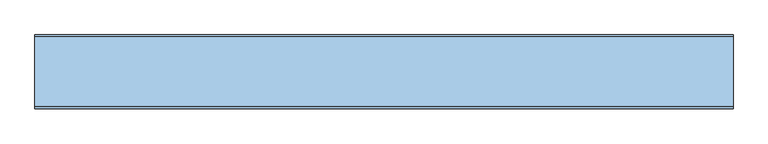
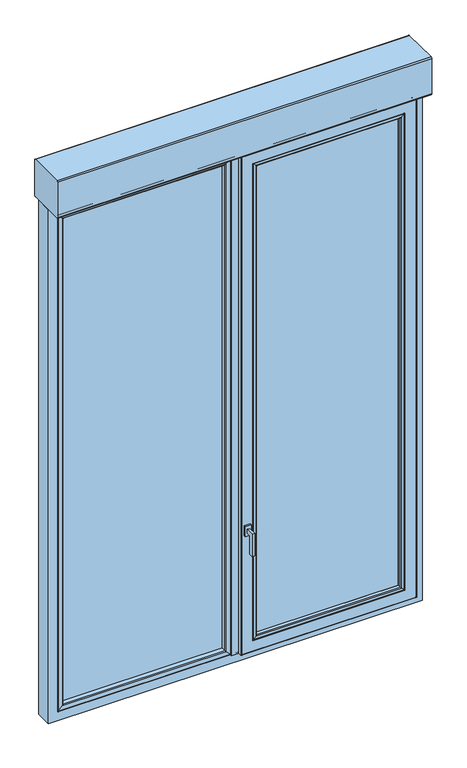
"""IFC4 building model written with IfcOpenShell, lengths in millimetres: window geometry, 2019_ES_Ventana_Replus_re80pvc301_11103_box_1-Hoja_Panel-Fijo-Lateral_con-Compacto : Salla."""

from ifc_helpers import new_model, si_unit, point, frame, frame_2d, origin, place, context, project, spatial, polyline, circle_curve, ellipse_curve, trimmed, segment, composite_curve, outline, extrude, source, transform, mapped, element, save
from ifc_brep_helpers import plane_surface, cylinder_surface, advanced_brep


def window_06f9a558(model_context):
    return source(origin(), model_context, "Body", "SolidModel", [
        extrude(outline(composite_curve([segment(polyline([(55.0, 3355.0), (-120.0, 3355.0)]), True, "CONTINUOUS"), segment(trimmed(circle_curve(frame_2d((-120.0, 3360.0)), 5.0), [point((-120.0, 3355.0))], [point((-125.0, 3360.0))], False, "CARTESIAN"), True, "CONTINUOUS"), segment(polyline([(-125.0, 3360.0), (-125.0, 3535.0)]), True, "CONTINUOUS"), segment(trimmed(circle_curve(frame_2d((-120.0, 3535.0)), 5.0), [point((-125.0, 3535.0))], [point((-120.0, 3540.0))], False, "CARTESIAN"), True, "CONTINUOUS"), segment(polyline([(-120.0, 3540.0), (55.0, 3540.0)]), True, "CONTINUOUS"), segment(trimmed(circle_curve(frame_2d((55.0, 3535.0)), 5.0), [point((55.0, 3540.0))], [point((60.0, 3535.0))], False, "CARTESIAN"), True, "CONTINUOUS"), segment(polyline([(60.0, 3535.0), (60.0, 3360.0)]), True, "CONTINUOUS"), segment(trimmed(circle_curve(frame_2d((55.0, 3360.0)), 5.0), [point((60.0, 3360.0))], [point((55.0, 3355.0))], False, "CARTESIAN"), True, "CONTINUOUS")], self_intersect=False)), frame((-875.0, 0.0, 0.0), z_axis=(1.0, 0.0, 0.0), x_axis=(0.0, 1.0, 0.0)), (0.0, 0.0, 1.0), 1750.0),
        extrude(outline(polyline([(-78.4999991, 1470.0), (-78.4999991, 1450.0), (-98.4999991, 1450.0), (-98.4999991, 1360.0), (-118.4999991, 1360.0), (-118.4999991, 1470.0), (-78.4999991, 1470.0)])), frame((38.5, 0.0, 0.0), z_axis=(1.0, 0.0, 0.0), x_axis=(0.0, 1.0, 0.0)), (0.0, 0.0, 1.0), 12.0),
        extrude(outline(polyline([(58.7312385, -78.4999991), (30.2687615, -78.4999991), (30.2687615, -68.4999991), (58.7312385, -68.4999991), (58.7312385, -78.4999991)])), frame((0.0, 0.0, 1435.217127), z_axis=(0.0, 0.0, 1.0), x_axis=(1.0, 0.0, 0.0)), (0.0, 0.0, 1.0), 49.565746),
        extrude(outline(polyline([(-37.0063666, 11.4999962), (-37.0063666, 7.4999962), (-809.1891471, 7.4999962), (-809.1891471, 11.4999962), (-37.0063666, 11.4999962)])), frame((0.0, 0.0, 875.6108529), z_axis=(0.0, 0.0, 1.0), x_axis=(1.0, 0.0, 0.0)), (0.0, 0.0, 1.0), 2413.7782941),
        extrude(outline(polyline([(-37.0063666, -6.5), (-37.0063666, -10.5), (-809.1891471, -10.5), (-809.1891471, -6.5), (-37.0063666, -6.5)])), frame((0.0, 0.0, 875.6108529), z_axis=(0.0, 0.0, 1.0), x_axis=(1.0, 0.0, 0.0)), (0.0, 0.0, 1.0), 2413.7782941),
        extrude(outline(polyline([(-37.0063666, -24.4999997), (-37.0063666, -28.4999997), (-809.1891471, -28.4999997), (-809.1891471, -24.4999997), (-37.0063666, -24.4999997)])), frame((0.0, 0.0, 875.6108529), z_axis=(0.0, 0.0, 1.0), x_axis=(1.0, 0.0, 0.0)), (0.0, 0.0, 1.0), 2413.7782941),
        advanced_brep(
        [(-22.1502489, -49.9816666, 3309.0497511), (-41.8192398, -49.2838062, 3289.3807602), (-41.8192398, -49.2838062, 875.6192398), (-22.1502489, -49.9816666, 855.9502489), (-46.4697163, -45.5846502, 3284.7302837), (-46.4697163, -45.5846502, 880.2697163), (-809.3807594, -49.2838062, 875.6192398), (-829.0497503, -49.9816666, 855.9502489), (-21.0, -48.871505, 3310.2), (-21.0, -48.871505, 854.8), (-51.0475336, -28.5000036, 3280.1524664), (-51.0475336, -28.5000036, 884.8475336), (-804.7302829, -45.5846502, 880.2697163), (-43.2922784, -28.5000036, 877.0922784), (-807.9077208, -28.5000036, 877.0922784), (-807.9077208, -28.5000036, 3287.9077216), (-43.2922784, -28.5000036, 3287.9077216), (-800.1524657, -28.5000036, 3280.1524664), (-800.1524657, -28.5000036, 884.8475336), (-35.4855, -36.306782, 3295.7145), (-35.4855, -36.306782, 869.2855), (-35.4855, -39.5069121, 3295.7145), (-35.4855, -39.5069121, 869.2855), (-815.7144993, -36.306782, 869.2855), (-21.0, -39.5069121, 854.8), (-830.1999993, -39.5069121, 854.8), (-830.1999993, -39.5069121, 3310.2), (-21.0, -39.5069121, 3310.2), (-815.7144993, -39.5069121, 3295.7145), (-815.7144993, -39.5069121, 869.2855), (-830.1999993, -48.871505, 854.8), (-809.3807594, -49.2838062, 3289.3807602), (-829.0497503, -49.9816666, 3309.0497511), (-804.7302829, -45.5846502, 3284.7302837), (-815.7144993, -36.306782, 3295.7145), (-830.1999993, -48.871505, 3310.2)],
        [
            (0, 1),
            (1, 2),
            (2, 3),
            (3, 0),
            (1, 4, ellipse_curve(frame((-41.6449168, -44.2918491, 3289.5550832), z_axis=(0.7071067811865475, 0.0, -0.7071067811865475), x_axis=(0.7071067811865474, 0.0, 0.7071067811865476)), 7.0639967, 4.995)),
            (4, 5),
            (5, 2, ellipse_curve(frame((-41.6449168, -44.2918491, 875.4449168), z_axis=(0.7071067811865475, 0.0, 0.7071067811865475), x_axis=(-0.7071067811865474, 0.0, 0.7071067811865476)), 7.0639967, 4.995)),
            (2, 6),
            (6, 7),
            (7, 3),
            (8, 0, ellipse_curve(frame((-22.1108601, -48.871505, 3309.0891399), z_axis=(0.7071067811865475, 0.0, -0.7071067811865475), x_axis=(0.7071067811865474, 0.0, 0.7071067811865476)), 1.5709935, 1.1108601)),
            (3, 9, ellipse_curve(frame((-22.1108601, -48.871505, 855.9108601), z_axis=(0.7071067811865475, 0.0, 0.7071067811865475), x_axis=(-0.7071067811865474, 0.0, 0.7071067811865476)), 1.5709935, 1.1108601)),
            (9, 8),
            (4, 10),
            (10, 11),
            (11, 5),
            (5, 12),
            (12, 6, ellipse_curve(frame((-809.5550824, -44.2918491, 875.4449168), z_axis=(0.7071067811865475, 0.0, -0.7071067811865475), x_axis=(0.7071067811865476, 0.0, 0.7071067811865474)), 7.0639967, 4.995)),
            (13, 14),
            (14, 15),
            (15, 16),
            (16, 13),
            (10, 17),
            (17, 18),
            (18, 11),
            (18, 12),
            (16, 19),
            (19, 20),
            (20, 13),
            (19, 21),
            (21, 22),
            (22, 20),
            (20, 23),
            (23, 14),
            (24, 25),
            (25, 26),
            (26, 27),
            (27, 24),
            (21, 28),
            (28, 29),
            (29, 22),
            (29, 23),
            (9, 24),
            (27, 8),
            (9, 30),
            (30, 25),
            (7, 30, ellipse_curve(frame((-829.0891391, -48.871505, 855.9108601), z_axis=(0.7071067811865475, 0.0, -0.7071067811865475), x_axis=(0.7071067811865476, 0.0, 0.7071067811865474)), 1.5709935, 1.1108601)),
            (6, 31),
            (31, 32),
            (32, 7),
            (12, 33),
            (33, 31, ellipse_curve(frame((-809.5550824, -44.2918491, 3289.5550832), z_axis=(-0.7071067811865475, 0.0, -0.7071067811865475), x_axis=(0.7071067811865474, 0.0, -0.7071067811865476)), 7.0639967, 4.995)),
            (17, 33),
            (23, 34),
            (34, 15),
            (28, 34),
            (30, 35),
            (35, 26),
            (32, 35, ellipse_curve(frame((-829.0891391, -48.871505, 3309.0891399), z_axis=(-0.7071067811865475, 0.0, -0.7071067811865475), x_axis=(0.7071067811865474, 0.0, -0.7071067811865476)), 1.5709935, 1.1108601)),
            (31, 1),
            (0, 32),
            (33, 4),
            (34, 19),
            (35, 8),
        ],
        [
            plane_surface(frame((-41.8192398, -49.2838062, 3289.3807602), z_axis=(-0.03545791932093311, -0.9993711702652975, 0.0), x_axis=(0.0, 0.0, -1.0))),
            cylinder_surface(frame((-41.6449168, -44.2918491, 3317.2), z_axis=(0.0, 0.0, 1.0), x_axis=(-1.0, 0.0, 0.0)), 4.995),
            plane_surface(frame((-41.8192398, -49.2838062, 875.6192398), z_axis=(0.0, -0.9993711702652976, 0.035457919320929884), x_axis=(-1.0, 0.0, 0.0))),
            cylinder_surface(frame((-22.1108601, -48.871505, 3317.2), z_axis=(0.0, 0.0, 1.0), x_axis=(-1.0, 0.0, 0.0)), 1.1108601),
            plane_surface(frame((-51.0475336, -28.5000036, 3280.1524664), z_axis=(-0.9659258262890619, -0.25881904510254483, 0.0), x_axis=(0.0, 0.0, -1.0))),
            cylinder_surface(frame((-14.0, -44.2918491, 875.4449168), z_axis=(1.0, 0.0, 0.0), x_axis=(0.0, 0.0, 1.0)), 4.995),
            plane_surface(frame((-807.9077208, -28.5000036, 3287.9077216), z_axis=(0.0, 1.0, 0.0), x_axis=(1.0, 0.0, 0.0))),
            plane_surface(frame((-51.0475336, -28.5000036, 884.8475336), z_axis=(0.0, -0.25881904510254794, 0.965925826289061), x_axis=(-1.0, 0.0, 0.0))),
            plane_surface(frame((-35.4855, -36.306782, 3295.7145), z_axis=(0.7071067811865617, 0.7071067811865334, 0.0), x_axis=(0.0, 0.0, -1.0))),
            plane_surface(frame((-35.4855, -39.5069121, 3295.7145), z_axis=(1.0, 0.0, 0.0), x_axis=(0.0, 0.0, -1.0))),
            plane_surface(frame((-35.4855, -36.306782, 869.2855), z_axis=(0.0, 0.7071067811865357, -0.7071067811865593), x_axis=(-1.0, 0.0, 0.0))),
            plane_surface(frame((-830.1999993, -39.5069121, 3310.2), z_axis=(0.0, 1.0, 0.0), x_axis=(1.0, 0.0, 0.0))),
            plane_surface(frame((-35.4855, -39.5069121, 869.2855), z_axis=(0.0, 0.0, -1.0), x_axis=(-1.0, 0.0, 0.0))),
            plane_surface(frame((-21.0, -46.2002121, 3310.2), z_axis=(1.0, 0.0, 0.0), x_axis=(0.0, 0.0, -1.0))),
            plane_surface(frame((-21.0, -46.2002121, 854.8), z_axis=(0.0, 0.0, -1.0), x_axis=(-1.0, 0.0, 0.0))),
            cylinder_surface(frame((-14.0, -48.871505, 855.9108601), z_axis=(1.0, 0.0, 0.0), x_axis=(0.0, 0.0, 1.0)), 1.1108601),
            plane_surface(frame((-809.3807594, -49.2838062, 875.6192398), z_axis=(0.03545791932092666, -0.9993711702652978, 0.0), x_axis=(0.0, 0.0, 1.0))),
            cylinder_surface(frame((-809.5550824, -44.2918491, 847.8), z_axis=(0.0, 0.0, -1.0), x_axis=(1.0, 0.0, 0.0)), 4.995),
            plane_surface(frame((-800.1524657, -28.5000036, 884.8475336), z_axis=(0.9659258262890602, -0.2588190451025511, 0.0), x_axis=(0.0, 0.0, 1.0))),
            plane_surface(frame((-815.7144993, -36.306782, 869.2855), z_axis=(-0.707106781186557, 0.707106781186538, 0.0), x_axis=(0.0, 0.0, 1.0))),
            plane_surface(frame((-815.7144993, -39.5069121, 869.2855), z_axis=(-1.0, 0.0, 0.0), x_axis=(0.0, 0.0, 1.0))),
            plane_surface(frame((-830.1999993, -46.2002121, 854.8), z_axis=(-1.0, 0.0, 0.0), x_axis=(0.0, 0.0, 1.0))),
            cylinder_surface(frame((-829.0891391, -48.871505, 847.8), z_axis=(0.0, 0.0, -1.0), x_axis=(1.0, 0.0, 0.0)), 1.1108601),
            plane_surface(frame((-809.3807594, -49.2838062, 3289.3807602), z_axis=(0.0, -0.9993711702652976, -0.035457919320929884), x_axis=(1.0, 0.0, 0.0))),
            cylinder_surface(frame((-837.1999993, -44.2918491, 3289.5550832), z_axis=(-1.0, 0.0, 0.0), x_axis=(0.0, 0.0, -1.0)), 4.995),
            plane_surface(frame((-800.1524657, -28.5000036, 3280.1524664), z_axis=(0.0, -0.258819045102548, -0.9659258262890611), x_axis=(1.0, 0.0, 0.0))),
            plane_surface(frame((-815.7144993, -36.306782, 3295.7145), z_axis=(0.0, 0.7071067811865357, 0.7071067811865593), x_axis=(1.0, 0.0, 0.0))),
            plane_surface(frame((-815.7144993, -39.5069121, 3295.7145), z_axis=(0.0, 0.0, 1.0), x_axis=(1.0, 0.0, 0.0))),
            plane_surface(frame((-830.1999993, -46.2002121, 3310.2), z_axis=(0.0, 0.0, 1.0), x_axis=(1.0, 0.0, 0.0))),
            cylinder_surface(frame((-837.1999993, -48.871505, 3309.0891399), z_axis=(-1.0, 0.0, 0.0), x_axis=(0.0, 0.0, -1.0)), 1.1108601),
        ],
        [
            (0, [[1, 2, 3, 4]]),
            (1, [[5, 6, 7, -2]]),
            (2, [[-3, 8, 9, 10]]),
            (3, [[11, -4, 12, 13]]),
            (4, [[14, 15, 16, -6]]),
            (5, [[-7, 17, 18, -8]]),
            (6, [[19, 20, 21, 22], [23, 24, 25, -15]]),
            (7, [[-16, -25, 26, -17]]),
            (8, [[27, 28, 29, -22]]),
            (9, [[30, 31, 32, -28]]),
            (10, [[-29, 33, 34, -19]]),
            (11, [[35, 36, 37, 38], [39, 40, 41, -31]]),
            (12, [[-32, -41, 42, -33]]),
            (13, [[-13, 43, -38, 44]]),
            (14, [[-43, 45, 46, -35]]),
            (15, [[-12, -10, 47, -45]]),
            (16, [[-9, 48, 49, 50]]),
            (17, [[-18, 51, 52, -48]]),
            (18, [[-26, -24, 53, -51]]),
            (19, [[-34, 54, 55, -20]]),
            (20, [[-42, -40, 56, -54]]),
            (21, [[-46, 57, 58, -36]]),
            (22, [[-47, -50, 59, -57]]),
            (23, [[-49, 60, -1, 61]]),
            (24, [[-52, 62, -5, -60]]),
            (25, [[-53, -23, -14, -62]]),
            (26, [[-55, 63, -27, -21]]),
            (27, [[-56, -39, -30, -63]]),
            (28, [[-58, 64, -44, -37]]),
            (29, [[-59, -61, -11, -64]]),
        ],
    ),
        extrude(outline(polyline([(3252.0, 772.1999993), (3252.0, 81.0), (912.8, 81.0), (912.8, 772.1999993), (3252.0, 772.1999993)]), holes=[polyline([(920.8, 764.1999993), (920.8, 89.0), (3244.0, 89.0), (3244.0, 764.1999993), (920.8, 764.1999993)])]), frame((0.0, -27.0000002, 0.0), z_axis=(0.0, 1.0, 0.0), x_axis=(0.0, 0.0, 1.0)), (0.0, 0.0, 1.0), 16.0000002),
        extrude(outline(polyline([(3252.0, 772.1999993), (3252.0, 81.0), (912.8, 81.0), (912.8, 772.1999993), (3252.0, 772.1999993)]), holes=[polyline([(920.8, 764.1999993), (920.8, 89.0), (3244.0, 89.0), (3244.0, 764.1999993), (920.8, 764.1999993)])]), frame((0.0, -47.0000002, 0.0), z_axis=(0.0, 1.0, 0.0), x_axis=(0.0, 0.0, 1.0)), (0.0, 0.0, 1.0), 16.0000002),
        extrude(outline(polyline([(3283.3891471, -43.0063666), (3283.3891471, -803.1891471), (881.8608529, -803.1891471), (881.8608529, -43.0063666), (3283.3891471, -43.0063666)]), holes=[polyline([(889.8608529, -51.0063666), (889.8608529, -795.1891471), (3275.3891471, -795.1891471), (3275.3891471, -51.0063666), (889.8608529, -51.0063666)])]), frame((0.0, -24.5, 0.0), z_axis=(0.0, 1.0, 0.0), x_axis=(0.0, 0.0, 1.0)), (0.0, 0.0, 1.0), 14.0),
        extrude(outline(polyline([(3283.3891471, -43.0063666), (3283.3891471, -803.1891471), (881.8608529, -803.1891471), (881.8608529, -43.0063666), (3283.3891471, -43.0063666)]), holes=[polyline([(889.8608529, -51.0063666), (889.8608529, -795.1891471), (3275.3891471, -795.1891471), (3275.3891471, -51.0063666), (889.8608529, -51.0063666)])]), frame((0.0, -6.5, 0.0), z_axis=(0.0, 1.0, 0.0), x_axis=(0.0, 0.0, 1.0)), (0.0, 0.0, 1.0), 14.0),
        advanced_brep(
        [(48.1911809, 11.5, 3285.2), (48.1911809, 11.5, 879.8), (48.1911809, -11.9999991, 879.8), (48.1911809, -11.9999991, 3285.2), (805.1999993, 11.5, 3285.2), (805.1999993, 11.5, 879.8), (88.2020856, 11.5, 919.8109047), (765.1890945, 11.5, 919.8109047), (765.1890945, 11.5, 3245.1890953), (88.2020856, 11.5, 3245.1890953), (805.1999993, -11.9999991, 879.8), (35.1911809, -11.9999991, 3298.2), (818.1999993, -11.9999991, 3298.2), (818.1999993, -11.9999991, 866.8), (35.1911809, -11.9999991, 866.8), (805.1999993, -11.9999991, 3285.2), (35.1911809, -50.0, 866.8), (35.1911809, -50.0, 3298.2), (818.1999993, -50.0, 866.8), (15.1911809, -50.0, 3318.2), (838.1999993, -50.0, 3318.2), (838.1999993, -50.0, 846.8), (15.1911809, -50.0, 846.8), (818.1999993, -50.0, 3298.2), (15.1911809, -65.4999991, 3318.2), (15.1911809, -65.4999991, 846.8), (838.1999993, -65.4999991, 846.8), (18.1911809, -68.4999991, 3315.2), (18.1911809, -68.4999991, 849.8), (835.1999993, -68.4999991, 849.8), (835.1999993, -68.4999991, 3315.2), (70.9541209, -68.4999991, 3262.43706), (782.4370593, -68.4999991, 3262.43706), (782.4370593, -68.4999991, 902.56294), (70.9541209, -68.4999991, 902.56294), (72.1911809, -67.2629391, 3261.2), (72.1911809, -67.2629391, 903.8), (781.1999993, -67.2629391, 903.8), (72.7423375, -67.7951848, 3260.6488434), (72.7423375, -67.7951848, 904.3511566), (780.6488427, -67.7951848, 904.3511566), (85.7676831, -67.3403297, 3247.6234978), (85.7676831, -67.3403297, 917.3765022), (767.6234971, -67.3403297, 917.3765022), (89.4917884, -64.3780426, 3243.8993925), (89.4917884, -64.3780426, 921.1006075), (763.8993918, -64.3780426, 921.1006075), (92.8970803, -51.6693201, 3240.4941006), (92.8970803, -51.6693201, 924.5058994), (760.4940999, -51.6693201, 924.5058994), (92.3834932, -51.0000003, 3241.0076877), (92.3834932, -51.0000003, 923.9923123), (761.007687, -51.0000003, 923.9923123), (81.1911809, -51.0000003, 3252.2), (772.1999993, -51.0000003, 3252.2), (772.1999993, -51.0000003, 912.8), (81.1911809, -51.0000003, 912.8), (761.007687, -51.0000003, 3241.0076877), (81.1911809, -56.4999995, 3252.2), (81.1911809, -56.4999995, 912.8), (772.1999993, -56.4999995, 912.8), (69.1911809, -56.4999995, 3264.2), (784.1999993, -56.4999995, 3264.2), (784.1999993, -56.4999995, 900.8), (69.1911809, -56.4999995, 900.8), (772.1999993, -56.4999995, 3252.2), (69.1911809, -25.6153717, 3264.2), (69.1911809, -25.6153717, 900.8), (784.1999993, -25.6153717, 900.8), (66.574961, -6.9999997, 3266.8162199), (66.574961, -6.9999997, 898.1837801), (786.8162192, -6.9999997, 898.1837801), (786.8162192, -6.9999997, 3266.8162199), (87.1911809, -6.9999997, 3246.2), (766.1999993, -6.9999997, 3246.2), (766.1999993, -6.9999997, 918.8), (87.1911809, -6.9999997, 918.8), (87.1911809, -3.0000033, 3246.2), (87.1911809, -3.0000033, 918.8), (766.1999993, -3.0000033, 918.8), (766.1999993, -3.0000033, 3246.2), (93.7172496, -3.0000033, 3239.6739313), (759.6739305, -3.0000033, 3239.6739313), (759.6739305, -3.0000033, 925.3260687), (93.7172496, -3.0000033, 925.3260687), (94.2153834, -2.3508228, 3239.1757976), (94.2153834, -2.3508228, 925.8242024), (759.1757968, -2.3508228, 925.8242024), (91.0998631, 9.2764571, 3242.2913178), (91.0998631, 9.2764571, 922.7086822), (762.2913171, 9.2764571, 922.7086822), (838.1999993, -65.4999991, 3318.2), (781.1999993, -67.2629391, 3261.2), (780.6488427, -67.7951848, 3260.6488434), (767.6234971, -67.3403297, 3247.6234978), (763.8993918, -64.3780426, 3243.8993925), (760.4940999, -51.6693201, 3240.4941006), (784.1999993, -25.6153717, 3264.2), (759.1757968, -2.3508228, 3239.1757976), (762.2913171, 9.2764571, 3242.2913178)],
        [
            (0, 1),
            (1, 2),
            (2, 3),
            (3, 0),
            (0, 4),
            (4, 5),
            (5, 1),
            (6, 7),
            (7, 8),
            (8, 9),
            (9, 6),
            (5, 10),
            (10, 2),
            (11, 12),
            (12, 13),
            (13, 14),
            (14, 11),
            (10, 15),
            (15, 3),
            (14, 16),
            (16, 17),
            (17, 11),
            (13, 18),
            (18, 16),
            (19, 20),
            (20, 21),
            (21, 22),
            (22, 19),
            (18, 23),
            (23, 17),
            (24, 19),
            (22, 25),
            (25, 24),
            (21, 26),
            (26, 25),
            (27, 24, ellipse_curve(frame((18.1911809, -65.4999991, 3315.2), z_axis=(-0.7071067811865475, 0.0, -0.7071067811865475), x_axis=(-0.7071067811865474, 0.0, 0.7071067811865476)), 4.2426407, 3.0)),
            (25, 28, ellipse_curve(frame((18.1911809, -65.4999991, 849.8), z_axis=(-0.7071067811865475, 0.0, 0.7071067811865475), x_axis=(0.7071067811865474, 0.0, 0.7071067811865476)), 4.2426407, 3.0)),
            (28, 27),
            (26, 29, ellipse_curve(frame((835.1999993, -65.4999991, 849.8), z_axis=(-0.7071067811865475, 0.0, -0.7071067811865475), x_axis=(-0.7071067811865476, 0.0, 0.7071067811865474)), 4.2426407, 3.0)),
            (29, 28),
            (29, 30),
            (30, 27),
            (31, 32),
            (32, 33),
            (33, 34),
            (34, 31),
            (35, 31, ellipse_curve(frame((70.9541209, -67.2629391, 3262.43706), z_axis=(-0.7071067811865475, 0.0, -0.7071067811865475), x_axis=(-0.7071067811865474, 0.0, 0.7071067811865476)), 1.7494671, 1.23706)),
            (34, 36, ellipse_curve(frame((70.9541209, -67.2629391, 902.56294), z_axis=(-0.7071067811865475, 0.0, 0.7071067811865475), x_axis=(0.7071067811865474, 0.0, 0.7071067811865476)), 1.7494671, 1.23706)),
            (36, 35),
            (33, 37, ellipse_curve(frame((782.4370593, -67.2629391, 902.56294), z_axis=(-0.7071067811865475, 0.0, -0.7071067811865475), x_axis=(-0.7071067811865476, 0.0, 0.7071067811865474)), 1.7494671, 1.23706)),
            (37, 36),
            (38, 35, ellipse_curve(frame((72.7237511, -67.2629391, 3260.6674299), z_axis=(-0.7071067811865475, 0.0, -0.7071067811865475), x_axis=(-0.7071067811865474, 0.0, 0.7071067811865476)), 0.7531679, 0.5325701)),
            (36, 39, ellipse_curve(frame((72.7237511, -67.2629391, 904.3325701), z_axis=(-0.7071067811865475, 0.0, 0.7071067811865475), x_axis=(0.7071067811865474, 0.0, 0.7071067811865476)), 0.7531679, 0.5325701)),
            (39, 38),
            (37, 40, ellipse_curve(frame((780.6674291, -67.2629391, 904.3325701), z_axis=(-0.7071067811865475, 0.0, -0.7071067811865475), x_axis=(-0.7071067811865476, 0.0, 0.7071067811865474)), 0.7531679, 0.5325701)),
            (40, 39),
            (41, 38),
            (39, 42),
            (42, 41),
            (40, 43),
            (43, 42),
            (44, 41, ellipse_curve(frame((85.6280851, -63.3427664, 3247.7630958), z_axis=(-0.7071067811865475, 0.0, -0.7071067811865475), x_axis=(-0.7071067811865474, 0.0, 0.7071067811865476)), 5.6568542, 4.0)),
            (42, 45, ellipse_curve(frame((85.6280851, -63.3427664, 917.2369042), z_axis=(-0.7071067811865475, 0.0, 0.7071067811865475), x_axis=(0.7071067811865474, 0.0, 0.7071067811865476)), 5.6568542, 4.0)),
            (45, 44),
            (43, 46, ellipse_curve(frame((767.7630951, -63.3427664, 917.2369042), z_axis=(-0.7071067811865475, 0.0, -0.7071067811865475), x_axis=(-0.7071067811865476, 0.0, 0.7071067811865474)), 5.6568542, 4.0)),
            (46, 45),
            (47, 44),
            (45, 48),
            (48, 47),
            (46, 49),
            (49, 48),
            (50, 47, ellipse_curve(frame((92.3834932, -51.5317048, 3241.0076877), z_axis=(-0.7071067811865475, 0.0, -0.7071067811865475), x_axis=(-0.7071067811865474, 0.0, 0.7071067811865476)), 0.7519437, 0.5317045)),
            (48, 51, ellipse_curve(frame((92.3834932, -51.5317048, 923.9923123), z_axis=(-0.7071067811865475, 0.0, 0.7071067811865475), x_axis=(0.7071067811865474, 0.0, 0.7071067811865476)), 0.7519437, 0.5317045)),
            (51, 50),
            (49, 52, ellipse_curve(frame((761.007687, -51.5317048, 923.9923123), z_axis=(-0.7071067811865475, 0.0, -0.7071067811865475), x_axis=(-0.7071067811865476, 0.0, 0.7071067811865474)), 0.7519437, 0.5317045)),
            (52, 51),
            (53, 54),
            (54, 55),
            (55, 56),
            (56, 53),
            (52, 57),
            (57, 50),
            (58, 53),
            (56, 59),
            (59, 58),
            (55, 60),
            (60, 59),
            (61, 62),
            (62, 63),
            (63, 64),
            (64, 61),
            (60, 65),
            (65, 58),
            (66, 61),
            (64, 67),
            (67, 66),
            (63, 68),
            (68, 67),
            (69, 66),
            (67, 70),
            (70, 69),
            (68, 71),
            (71, 70),
            (71, 72),
            (72, 69),
            (73, 74),
            (74, 75),
            (75, 76),
            (76, 73),
            (77, 73),
            (76, 78),
            (78, 77),
            (75, 79),
            (79, 78),
            (79, 80),
            (80, 77),
            (81, 82),
            (82, 83),
            (83, 84),
            (84, 81),
            (85, 81, ellipse_curve(frame((93.7172496, -2.4842973, 3239.6739313), z_axis=(-0.7071067811865475, 0.0, -0.7071067811865475), x_axis=(-0.7071067811865474, 0.0, 0.7071067811865476)), 0.7293184, 0.515706)),
            (84, 86, ellipse_curve(frame((93.7172496, -2.4842973, 925.3260687), z_axis=(-0.7071067811865475, 0.0, 0.7071067811865475), x_axis=(0.7071067811865474, 0.0, 0.7071067811865476)), 0.7293184, 0.515706)),
            (86, 85),
            (83, 87, ellipse_curve(frame((759.6739305, -2.4842973, 925.3260687), z_axis=(-0.7071067811865475, 0.0, -0.7071067811865475), x_axis=(-0.7071067811865476, 0.0, 0.7071067811865474)), 0.7293184, 0.515706)),
            (87, 86),
            (88, 85),
            (86, 89),
            (89, 88),
            (87, 90),
            (90, 89),
            (9, 88, ellipse_curve(frame((88.2020856, 8.5, 3245.1890953), z_axis=(-0.7071067811865475, 0.0, -0.7071067811865475), x_axis=(-0.7071067811865474, 0.0, 0.7071067811865476)), 4.2426407, 3.0)),
            (89, 6, ellipse_curve(frame((88.2020856, 8.5, 919.8109047), z_axis=(-0.7071067811865475, 0.0, 0.7071067811865475), x_axis=(0.7071067811865474, 0.0, 0.7071067811865476)), 4.2426407, 3.0)),
            (90, 7, ellipse_curve(frame((765.1890945, 8.5, 919.8109047), z_axis=(-0.7071067811865475, 0.0, -0.7071067811865475), x_axis=(-0.7071067811865476, 0.0, 0.7071067811865474)), 4.2426407, 3.0)),
            (4, 15),
            (12, 23),
            (20, 91),
            (91, 26),
            (91, 30, ellipse_curve(frame((835.1999993, -65.4999991, 3315.2), z_axis=(0.7071067811865475, 0.0, -0.7071067811865475), x_axis=(-0.7071067811865474, 0.0, -0.7071067811865476)), 4.2426407, 3.0)),
            (32, 92, ellipse_curve(frame((782.4370593, -67.2629391, 3262.43706), z_axis=(0.7071067811865475, 0.0, -0.7071067811865475), x_axis=(-0.7071067811865474, 0.0, -0.7071067811865476)), 1.7494671, 1.23706)),
            (92, 37),
            (92, 93, ellipse_curve(frame((780.6674291, -67.2629391, 3260.6674299), z_axis=(0.7071067811865475, 0.0, -0.7071067811865475), x_axis=(-0.7071067811865474, 0.0, -0.7071067811865476)), 0.7531679, 0.5325701)),
            (93, 40),
            (93, 94),
            (94, 43),
            (94, 95, ellipse_curve(frame((767.7630951, -63.3427664, 3247.7630958), z_axis=(0.7071067811865475, 0.0, -0.7071067811865475), x_axis=(-0.7071067811865474, 0.0, -0.7071067811865476)), 5.6568542, 4.0)),
            (95, 46),
            (95, 96),
            (96, 49),
            (96, 57, ellipse_curve(frame((761.007687, -51.5317048, 3241.0076877), z_axis=(0.7071067811865475, 0.0, -0.7071067811865475), x_axis=(-0.7071067811865474, 0.0, -0.7071067811865476)), 0.7519437, 0.5317045)),
            (54, 65),
            (62, 97),
            (97, 68),
            (97, 72),
            (74, 80),
            (82, 98, ellipse_curve(frame((759.6739305, -2.4842973, 3239.6739313), z_axis=(0.7071067811865475, 0.0, -0.7071067811865475), x_axis=(-0.7071067811865474, 0.0, -0.7071067811865476)), 0.7293184, 0.515706)),
            (98, 87),
            (98, 99),
            (99, 90),
            (99, 8, ellipse_curve(frame((765.1890945, 8.5, 3245.1890953), z_axis=(0.7071067811865475, 0.0, -0.7071067811865475), x_axis=(-0.7071067811865474, 0.0, -0.7071067811865476)), 4.2426407, 3.0)),
            (24, 91),
            (35, 92),
            (38, 93),
            (41, 94),
            (44, 95),
            (47, 96),
            (66, 97),
            (85, 98),
            (88, 99),
        ],
        [
            plane_surface(frame((48.1911809, -1.4999991, 3285.2), z_axis=(-1.0, 0.0, 0.0), x_axis=(0.0, 0.0, -1.0))),
            plane_surface(frame((765.1890945, 11.5, 3245.1890953), z_axis=(0.0, 1.0, 0.0), x_axis=(-1.0, 0.0, 0.0))),
            plane_surface(frame((48.1911809, -1.4999991, 879.8), z_axis=(0.0, 0.0, -1.0), x_axis=(1.0, 0.0, 0.0))),
            plane_surface(frame((810.7000002, -11.9999991, 3290.7000009), z_axis=(0.0, 1.0, 0.0), x_axis=(-1.0, 0.0, 0.0))),
            plane_surface(frame((35.1911809, -45.0999991, 3298.2), z_axis=(-1.0, 0.0, 0.0), x_axis=(0.0, 0.0, -1.0))),
            plane_surface(frame((35.1911809, -45.0999991, 866.8), z_axis=(0.0, 0.0, -1.0), x_axis=(1.0, 0.0, 0.0))),
            plane_surface(frame((834.2000019, -50.0, 3314.2000027), z_axis=(0.0, 1.0, 0.0), x_axis=(-1.0, 0.0, 0.0))),
            plane_surface(frame((15.1911809, -50.0, 3318.2), z_axis=(-1.0, 0.0, 0.0), x_axis=(0.0, 0.0, -1.0))),
            plane_surface(frame((15.1911809, -50.0, 846.8), z_axis=(0.0, 0.0, -1.0), x_axis=(1.0, 0.0, 0.0))),
            cylinder_surface(frame((18.1911809, -65.4999991, 3318.2), z_axis=(0.0, 0.0, 1.0), x_axis=(0.0, 1.0, 0.0)), 3.0),
            cylinder_surface(frame((15.1911809, -65.4999991, 849.8), z_axis=(-1.0, 0.0, 0.0), x_axis=(0.0, 1.0, 0.0)), 3.0),
            plane_surface(frame((835.1999993, -68.4999991, 3315.2), z_axis=(0.0, -1.0, 0.0), x_axis=(-1.0, 0.0, 0.0))),
            cylinder_surface(frame((70.9541209, -67.2629391, 3318.2), z_axis=(0.0, 0.0, 1.0), x_axis=(0.0, 1.0, 0.0)), 1.23706),
            cylinder_surface(frame((15.1911809, -67.2629391, 902.56294), z_axis=(-1.0, 0.0, 0.0), x_axis=(0.0, 1.0, 0.0)), 1.23706),
            cylinder_surface(frame((72.7237511, -67.2629391, 3318.2), z_axis=(0.0, 0.0, 1.0), x_axis=(0.0, 1.0, 0.0)), 0.5325701),
            cylinder_surface(frame((15.1911809, -67.2629391, 904.3325701), z_axis=(-1.0, 0.0, 0.0), x_axis=(0.0, 1.0, 0.0)), 0.5325701),
            plane_surface(frame((72.7423375, -67.7951848, 3260.6488434), z_axis=(0.03489949670249966, -0.9993908270190959, 0.0), x_axis=(0.0, 0.0, -1.0))),
            plane_surface(frame((72.7423375, -67.7951848, 904.3511566), z_axis=(0.0, -0.9993908270190958, 0.034899496702502884), x_axis=(1.0, 0.0, 0.0))),
            cylinder_surface(frame((85.6280851, -63.3427664, 3318.2), z_axis=(0.0, 0.0, 1.0), x_axis=(0.0, 1.0, 0.0)), 4.0),
            cylinder_surface(frame((15.1911809, -63.3427664, 917.2369042), z_axis=(-1.0, 0.0, 0.0), x_axis=(0.0, 1.0, 0.0)), 4.0),
            plane_surface(frame((89.4917884, -64.3780426, 3243.8993925), z_axis=(0.9659258262890643, -0.2588190451025359, 0.0), x_axis=(0.0, 0.0, -1.0))),
            plane_surface(frame((89.4917884, -64.3780426, 921.1006075), z_axis=(0.0, -0.2588190451025328, 0.9659258262890652), x_axis=(1.0, 0.0, 0.0))),
            cylinder_surface(frame((92.3834932, -51.5317048, 3318.2), z_axis=(0.0, 0.0, 1.0), x_axis=(0.0, 1.0, 0.0)), 0.5317045),
            cylinder_surface(frame((15.1911809, -51.5317048, 923.9923123), z_axis=(-1.0, 0.0, 0.0), x_axis=(0.0, 1.0, 0.0)), 0.5317045),
            plane_surface(frame((761.007687, -51.0000003, 3241.0076877), z_axis=(0.0, 1.0, 0.0), x_axis=(-1.0, 0.0, 0.0))),
            plane_surface(frame((81.1911809, -51.0000003, 3252.2), z_axis=(-1.0, 0.0, 0.0), x_axis=(0.0, 0.0, -1.0))),
            plane_surface(frame((81.1911809, -51.0000003, 912.8), z_axis=(0.0, 0.0, -1.0), x_axis=(1.0, 0.0, 0.0))),
            plane_surface(frame((772.1999993, -56.4999995, 3252.2), z_axis=(0.0, 1.0, 0.0), x_axis=(-1.0, 0.0, 0.0))),
            plane_surface(frame((69.1911809, -56.4999995, 3264.2), z_axis=(1.0, 0.0, 0.0), x_axis=(0.0, 0.0, -1.0))),
            plane_surface(frame((69.1911809, -56.4999995, 900.8), z_axis=(0.0, 0.0, 1.0), x_axis=(1.0, 0.0, 0.0))),
            plane_surface(frame((69.1911809, -25.6153717, 3264.2), z_axis=(0.9902680687415736, 0.13917310096004257, 0.0), x_axis=(0.0, 0.0, -1.0))),
            plane_surface(frame((69.1911809, -25.6153717, 900.8), z_axis=(0.0, 0.13917310096004576, 0.9902680687415731), x_axis=(1.0, 0.0, 0.0))),
            plane_surface(frame((786.8162192, -6.9999997, 3266.8162199), z_axis=(0.0, -1.0, 0.0), x_axis=(-1.0, 0.0, 0.0))),
            plane_surface(frame((87.1911809, -6.9999997, 3246.2), z_axis=(1.0, 0.0, 0.0), x_axis=(0.0, 0.0, -1.0))),
            plane_surface(frame((87.1911809, -6.9999997, 918.8), z_axis=(0.0, 0.0, 1.0), x_axis=(1.0, 0.0, 0.0))),
            plane_surface(frame((766.1999993, -3.0000033, 3246.2), z_axis=(0.0, -1.0, 0.0), x_axis=(-1.0, 0.0, 0.0))),
            cylinder_surface(frame((93.7172496, -2.4842973, 3318.2), z_axis=(0.0, 0.0, 1.0), x_axis=(0.0, 1.0, 0.0)), 0.515706),
            cylinder_surface(frame((15.1911809, -2.4842973, 925.3260687), z_axis=(-1.0, 0.0, 0.0), x_axis=(0.0, 1.0, 0.0)), 0.515706),
            plane_surface(frame((94.2153834, -2.3508228, 3239.1757976), z_axis=(0.9659258263570589, 0.2588190448487762, 0.0), x_axis=(0.0, 0.0, -1.0))),
            plane_surface(frame((94.2153834, -2.3508228, 925.8242024), z_axis=(0.0, 0.2588190448487794, 0.9659258263570581), x_axis=(1.0, 0.0, 0.0))),
            cylinder_surface(frame((88.2020856, 8.5, 3318.2), z_axis=(0.0, 0.0, 1.0), x_axis=(0.0, 1.0, 0.0)), 3.0),
            cylinder_surface(frame((15.1911809, 8.5, 919.8109047), z_axis=(-1.0, 0.0, 0.0), x_axis=(0.0, 1.0, 0.0)), 3.0),
            plane_surface(frame((805.1999993, -1.4999991, 879.8), z_axis=(1.0, 0.0, 0.0), x_axis=(0.0, 0.0, 1.0))),
            plane_surface(frame((818.1999993, -45.0999991, 866.8), z_axis=(1.0, 0.0, 0.0), x_axis=(0.0, 0.0, 1.0))),
            plane_surface(frame((838.1999993, -50.0, 846.8), z_axis=(1.0, 0.0, 0.0), x_axis=(0.0, 0.0, 1.0))),
            cylinder_surface(frame((835.1999993, -65.4999991, 846.8), z_axis=(0.0, 0.0, -1.0), x_axis=(0.0, 1.0, 0.0)), 3.0),
            cylinder_surface(frame((782.4370593, -67.2629391, 846.8), z_axis=(0.0, 0.0, -1.0), x_axis=(0.0, 1.0, 0.0)), 1.23706),
            cylinder_surface(frame((780.6674291, -67.2629391, 846.8), z_axis=(0.0, 0.0, -1.0), x_axis=(0.0, 1.0, 0.0)), 0.5325701),
            plane_surface(frame((780.6488427, -67.7951848, 904.3511566), z_axis=(-0.03489949670250611, -0.9993908270190957, 0.0), x_axis=(0.0, 0.0, 1.0))),
            cylinder_surface(frame((767.7630951, -63.3427664, 846.8), z_axis=(0.0, 0.0, -1.0), x_axis=(0.0, 1.0, 0.0)), 4.0),
            plane_surface(frame((763.8993918, -64.3780426, 921.1006075), z_axis=(-0.965925826289066, -0.2588190451025297, 0.0), x_axis=(0.0, 0.0, 1.0))),
            cylinder_surface(frame((761.007687, -51.5317048, 846.8), z_axis=(0.0, 0.0, -1.0), x_axis=(0.0, 1.0, 0.0)), 0.5317045),
            plane_surface(frame((772.1999993, -51.0000003, 912.8), z_axis=(1.0, 0.0, 0.0), x_axis=(0.0, 0.0, 1.0))),
            plane_surface(frame((784.1999993, -56.4999995, 900.8), z_axis=(-1.0, 0.0, 0.0), x_axis=(0.0, 0.0, 1.0))),
            plane_surface(frame((784.1999993, -25.6153717, 900.8), z_axis=(-0.9902680687415727, 0.13917310096004895, 0.0), x_axis=(0.0, 0.0, 1.0))),
            plane_surface(frame((766.1999993, -6.9999997, 918.8), z_axis=(-1.0, 0.0, 0.0), x_axis=(0.0, 0.0, 1.0))),
            cylinder_surface(frame((759.6739305, -2.4842973, 846.8), z_axis=(0.0, 0.0, -1.0), x_axis=(0.0, 1.0, 0.0)), 0.515706),
            plane_surface(frame((759.1757968, -2.3508228, 925.8242024), z_axis=(-0.9659258263570573, 0.2588190448487825, 0.0), x_axis=(0.0, 0.0, 1.0))),
            cylinder_surface(frame((765.1890945, 8.5, 846.8), z_axis=(0.0, 0.0, -1.0), x_axis=(0.0, 1.0, 0.0)), 3.0),
            plane_surface(frame((805.1999993, -1.4999991, 3285.2), z_axis=(0.0, 0.0, 1.0), x_axis=(-1.0, 0.0, 0.0))),
            plane_surface(frame((818.1999993, -45.0999991, 3298.2), z_axis=(0.0, 0.0, 1.0), x_axis=(-1.0, 0.0, 0.0))),
            plane_surface(frame((838.1999993, -50.0, 3318.2), z_axis=(0.0, 0.0, 1.0), x_axis=(-1.0, 0.0, 0.0))),
            cylinder_surface(frame((838.1999993, -65.4999991, 3315.2), z_axis=(1.0, 0.0, 0.0), x_axis=(0.0, 1.0, 0.0)), 3.0),
            cylinder_surface(frame((838.1999993, -67.2629391, 3262.43706), z_axis=(1.0, 0.0, 0.0), x_axis=(0.0, 1.0, 0.0)), 1.23706),
            cylinder_surface(frame((838.1999993, -67.2629391, 3260.6674299), z_axis=(1.0, 0.0, 0.0), x_axis=(0.0, 1.0, 0.0)), 0.5325701),
            plane_surface(frame((780.6488427, -67.7951848, 3260.6488434), z_axis=(0.0, -0.9993908270190958, -0.034899496702502884), x_axis=(-1.0, 0.0, 0.0))),
            cylinder_surface(frame((838.1999993, -63.3427664, 3247.7630958), z_axis=(1.0, 0.0, 0.0), x_axis=(0.0, 1.0, 0.0)), 4.0),
            plane_surface(frame((763.8993918, -64.3780426, 3243.8993925), z_axis=(0.0, -0.2588190451025328, -0.9659258262890651), x_axis=(-1.0, 0.0, 0.0))),
            cylinder_surface(frame((838.1999993, -51.5317048, 3241.0076877), z_axis=(1.0, 0.0, 0.0), x_axis=(0.0, 1.0, 0.0)), 0.5317045),
            plane_surface(frame((772.1999993, -51.0000003, 3252.2), z_axis=(0.0, 0.0, 1.0), x_axis=(-1.0, 0.0, 0.0))),
            plane_surface(frame((784.1999993, -56.4999995, 3264.2), z_axis=(0.0, 0.0, -1.0), x_axis=(-1.0, 0.0, 0.0))),
            plane_surface(frame((784.1999993, -25.6153717, 3264.2), z_axis=(0.0, 0.13917310096004576, -0.9902680687415731), x_axis=(-1.0, 0.0, 0.0))),
            plane_surface(frame((766.1999993, -6.9999997, 3246.2), z_axis=(0.0, 0.0, -1.0), x_axis=(-1.0, 0.0, 0.0))),
            cylinder_surface(frame((838.1999993, -2.4842973, 3239.6739313), z_axis=(1.0, 0.0, 0.0), x_axis=(0.0, 1.0, 0.0)), 0.515706),
            plane_surface(frame((759.1757968, -2.3508228, 3239.1757976), z_axis=(0.0, 0.2588190448487794, -0.9659258263570581), x_axis=(-1.0, 0.0, 0.0))),
            cylinder_surface(frame((838.1999993, 8.5, 3245.1890953), z_axis=(1.0, 0.0, 0.0), x_axis=(0.0, 1.0, 0.0)), 3.0),
        ],
        [
            (0, [[1, 2, 3, 4]]),
            (1, [[5, 6, 7, -1], [8, 9, 10, 11]]),
            (2, [[-2, -7, 12, 13]]),
            (3, [[14, 15, 16, 17], [-13, 18, 19, -3]]),
            (4, [[-17, 20, 21, 22]]),
            (5, [[-20, -16, 23, 24]]),
            (6, [[25, 26, 27, 28], [-24, 29, 30, -21]]),
            (7, [[31, -28, 32, 33]]),
            (8, [[-32, -27, 34, 35]]),
            (9, [[36, -33, 37, 38]]),
            (10, [[-37, -35, 39, 40]]),
            (11, [[-40, 41, 42, -38], [43, 44, 45, 46]]),
            (12, [[47, -46, 48, 49]]),
            (13, [[-48, -45, 50, 51]]),
            (14, [[52, -49, 53, 54]]),
            (15, [[-53, -51, 55, 56]]),
            (16, [[57, -54, 58, 59]]),
            (17, [[-58, -56, 60, 61]]),
            (18, [[62, -59, 63, 64]]),
            (19, [[-63, -61, 65, 66]]),
            (20, [[67, -64, 68, 69]]),
            (21, [[-68, -66, 70, 71]]),
            (22, [[72, -69, 73, 74]]),
            (23, [[-73, -71, 75, 76]]),
            (24, [[77, 78, 79, 80], [-76, 81, 82, -74]]),
            (25, [[83, -80, 84, 85]]),
            (26, [[-84, -79, 86, 87]]),
            (27, [[88, 89, 90, 91], [-87, 92, 93, -85]]),
            (28, [[94, -91, 95, 96]]),
            (29, [[-95, -90, 97, 98]]),
            (30, [[99, -96, 100, 101]]),
            (31, [[-100, -98, 102, 103]]),
            (32, [[-103, 104, 105, -101], [106, 107, 108, 109]]),
            (33, [[110, -109, 111, 112]]),
            (34, [[-111, -108, 113, 114]]),
            (35, [[-114, 115, 116, -112], [117, 118, 119, 120]]),
            (36, [[121, -120, 122, 123]]),
            (37, [[-122, -119, 124, 125]]),
            (38, [[126, -123, 127, 128]]),
            (39, [[-127, -125, 129, 130]]),
            (40, [[131, -128, 132, -11]]),
            (41, [[-132, -130, 133, -8]]),
            (42, [[-12, -6, 134, -18]]),
            (43, [[-23, -15, 135, -29]]),
            (44, [[-34, -26, 136, 137]]),
            (45, [[-39, -137, 138, -41]]),
            (46, [[-50, -44, 139, 140]]),
            (47, [[-55, -140, 141, 142]]),
            (48, [[-60, -142, 143, 144]]),
            (49, [[-65, -144, 145, 146]]),
            (50, [[-70, -146, 147, 148]]),
            (51, [[-75, -148, 149, -81]]),
            (52, [[-86, -78, 150, -92]]),
            (53, [[-97, -89, 151, 152]]),
            (54, [[-102, -152, 153, -104]]),
            (55, [[-113, -107, 154, -115]]),
            (56, [[-124, -118, 155, 156]]),
            (57, [[-129, -156, 157, 158]]),
            (58, [[-133, -158, 159, -9]]),
            (59, [[-134, -5, -4, -19]]),
            (60, [[-135, -14, -22, -30]]),
            (61, [[-136, -25, -31, 160]]),
            (62, [[-138, -160, -36, -42]]),
            (63, [[-139, -43, -47, 161]]),
            (64, [[-141, -161, -52, 162]]),
            (65, [[-143, -162, -57, 163]]),
            (66, [[-145, -163, -62, 164]]),
            (67, [[-147, -164, -67, 165]]),
            (68, [[-149, -165, -72, -82]]),
            (69, [[-150, -77, -83, -93]]),
            (70, [[-151, -88, -94, 166]]),
            (71, [[-153, -166, -99, -105]]),
            (72, [[-154, -106, -110, -116]]),
            (73, [[-155, -117, -121, 167]]),
            (74, [[-157, -167, -126, 168]]),
            (75, [[-159, -168, -131, -10]]),
        ],
    ),
        extrude(outline(composite_curve([segment(polyline([(23.3911809, -37.9746327), (23.3911809, -49.0)]), True, "CONTINUOUS"), segment(trimmed(circle_curve(frame_2d((22.3911809, -49.0)), 1.0), [point((23.3911809, -49.0))], [point((22.3911809, -50.0))], False, "CARTESIAN"), True, "CONTINUOUS"), segment(polyline([(22.3911809, -50.0), (-19.7446784, -50.0)]), True, "CONTINUOUS"), segment(trimmed(circle_curve(frame_2d((-19.7446784, -49.0)), 1.0), [point((-19.7446784, -50.0))], [point((-20.7446784, -49.0))], False, "CARTESIAN"), True, "CONTINUOUS"), segment(polyline([(-20.7446784, -49.0), (-20.7446784, -37.9746327), (-18.5911809, -37.9746327), (-18.5911809, -8.0), (-40.6020331, -8.0), (-40.6020331, -6.2175904), (-27.9799071, 1.0697975), (-26.7556588, 15.0630198), (-41.0115567, 17.0665556), (-41.7938856, 11.4999962), (-52.5579009, 11.4999962)]), True, "CONTINUOUS"), segment(trimmed(circle_curve(frame_2d((-52.5579009, 12.4999962)), 1.0), [point((-52.5579009, 11.4999962))], [point((-53.5238267, 12.7588152))], False, "CARTESIAN"), True, "CONTINUOUS"), segment(polyline([(-53.5238267, 12.7588152), (-49.4998617, 27.7764571)]), True, "CONTINUOUS"), segment(trimmed(circle_curve(frame_2d((-46.6020842, 27.0)), 3.0), [point((-49.4998617, 27.7764571))], [point((-46.6020842, 30.0))], False, "CARTESIAN"), True, "CONTINUOUS"), segment(polyline([(-46.6020842, 30.0), (48.4020842, 30.0)]), True, "CONTINUOUS"), segment(trimmed(circle_curve(frame_2d((48.4020842, 27.0)), 3.0), [point((48.4020842, 30.0))], [point((51.2998617, 27.7764571))], False, "CARTESIAN"), True, "CONTINUOUS"), segment(polyline([(51.2998617, 27.7764571), (55.3238267, 12.7588152)]), True, "CONTINUOUS"), segment(trimmed(circle_curve(frame_2d((54.3579009, 12.4999962)), 1.0), [point((55.3238267, 12.7588152))], [point((54.3579009, 11.4999962))], False, "CARTESIAN"), True, "CONTINUOUS"), segment(polyline([(54.3579009, 11.4999962), (43.5938856, 11.4999962), (42.8115567, 17.0665556), (28.5556588, 15.0630198), (29.7799071, 1.0697975), (42.4020331, -6.2175904), (42.4020331, -8.0), (20.3911809, -8.0), (20.3911809, -37.9746327), (23.3911809, -37.9746327)]), True, "CONTINUOUS")], self_intersect=False)), frame((0.0, 0.0, 846.8), z_axis=(0.0, 0.0, 1.0), x_axis=(1.0, 0.0, 0.0)), (0.0, 0.0, 1.0), 2471.4),
        extrude(outline(polyline([(778.1999993, -6.9999997), (778.1999993, -10.9999997), (75.0, -10.9999997), (75.0, -6.9999997), (778.1999993, -6.9999997)])), frame((0.0, 0.0, 906.8), z_axis=(0.0, 0.0, 1.0), x_axis=(1.0, 0.0, 0.0)), (0.0, 0.0, 1.0), 2351.2),
        extrude(outline(polyline([(778.1999993, -26.9999997), (778.1999993, -30.9999997), (75.0, -30.9999997), (75.0, -26.9999997), (778.1999993, -26.9999997)])), frame((0.0, 0.0, 906.8), z_axis=(0.0, 0.0, 1.0), x_axis=(1.0, 0.0, 0.0)), (0.0, 0.0, 1.0), 2351.2),
        extrude(outline(polyline([(778.1999993, -46.9999997), (778.1999993, -50.9999997), (75.0, -50.9999997), (75.0, -46.9999997), (778.1999993, -46.9999997)])), frame((0.0, 0.0, 906.8), z_axis=(0.0, 0.0, 1.0), x_axis=(1.0, 0.0, 0.0)), (0.0, 0.0, 1.0), 2351.2),
        advanced_brep(
        [(831.1999993, -50.0, 3311.1999993), (830.1999993, -49.0, 3310.1999993), (830.1999993, -49.0, 854.8000007), (831.1999993, -50.0, 853.8000007), (830.1999993, -8.0, 3310.1999993), (830.1999993, -8.0, 854.8000007), (-830.1999993, -49.0, 854.8000007), (-831.1999993, -50.0, 853.8000007), (875.0, -50.0, 3355.0), (-875.0, -50.0, 3355.0), (-875.0, -50.0, 810.0), (875.0, -50.0, 810.0), (-831.1999993, -50.0, 3311.1999993), (799.2332803, 11.5, 3279.2332803), (798.2673545, 12.758819, 3278.2673545), (798.2673545, 12.758819, 886.7326455), (799.2332803, 11.5, 885.7667197), (802.2913185, 27.7764571, 3282.2913185), (802.2913185, 27.7764571, 882.7086815), (-798.2673545, 12.758819, 886.7326455), (-799.2332803, 11.5, 885.7667197), (811.1891471, 11.5, 3291.1891471), (-811.1891471, 11.5, 3291.1891471), (-811.1891471, 11.5, 873.8108529), (811.1891471, 11.5, 873.8108529), (-799.2332803, 11.5, 3279.2332803), (805.189096, 30.0, 3285.189096), (805.189096, 30.0, 879.810904), (875.0, 30.0, 810.0), (-875.0, 30.0, 810.0), (-875.0, 30.0, 3355.0), (875.0, 30.0, 3355.0), (-805.189096, 30.0, 3285.189096), (-805.189096, 30.0, 879.810904), (-802.2913185, 27.7764571, 882.7086815), (811.1891471, -8.0, 3291.1891471), (811.1891471, -8.0, 873.8108529), (-811.1891471, -8.0, 873.8108529), (-830.1999993, -8.0, 3310.1999993), (-830.1999993, -8.0, 854.8000007), (-811.1891471, -8.0, 3291.1891471), (-830.1999993, -49.0, 3310.1999993), (-798.2673545, 12.758819, 3278.2673545), (-802.2913185, 27.7764571, 3282.2913185)],
        [
            (0, 1, ellipse_curve(frame((831.1999993, -49.0, 3311.1999993), z_axis=(0.7071067811865475, 0.0, -0.7071067811865475), x_axis=(0.7071067811865474, 0.0, 0.7071067811865476)), 1.4142136, 1.0)),
            (1, 2),
            (2, 3, ellipse_curve(frame((831.1999993, -49.0, 853.8000007), z_axis=(0.7071067811865475, 0.0, 0.7071067811865475), x_axis=(-0.7071067811865474, 0.0, 0.7071067811865476)), 1.4142136, 1.0)),
            (3, 0),
            (1, 4),
            (4, 5),
            (5, 2),
            (2, 6),
            (6, 7, ellipse_curve(frame((-831.1999993, -49.0, 853.8000007), z_axis=(0.7071067811865475, 0.0, -0.7071067811865475), x_axis=(0.7071067811865476, 0.0, 0.7071067811865474)), 1.4142136, 1.0)),
            (7, 3),
            (8, 9),
            (9, 10),
            (10, 11),
            (11, 8),
            (7, 12),
            (12, 0),
            (13, 14, ellipse_curve(frame((799.2332803, 12.5, 3279.2332803), z_axis=(0.7071067811865475, 0.0, -0.7071067811865475), x_axis=(0.7071067811865474, 0.0, 0.7071067811865476)), 1.4142136, 1.0)),
            (14, 15),
            (15, 16, ellipse_curve(frame((799.2332803, 12.5, 885.7667197), z_axis=(0.7071067811865475, 0.0, 0.7071067811865475), x_axis=(-0.7071067811865474, 0.0, 0.7071067811865476)), 1.4142136, 1.0)),
            (16, 13),
            (14, 17),
            (17, 18),
            (18, 15),
            (15, 19),
            (19, 20, ellipse_curve(frame((-799.2332803, 12.5, 885.7667197), z_axis=(0.7071067811865475, 0.0, -0.7071067811865475), x_axis=(0.7071067811865476, 0.0, 0.7071067811865474)), 1.4142136, 1.0)),
            (20, 16),
            (21, 22),
            (22, 23),
            (23, 24),
            (24, 21),
            (20, 25),
            (25, 13),
            (17, 26, ellipse_curve(frame((805.189096, 27.0, 3285.189096), z_axis=(0.7071067811865475, 0.0, -0.7071067811865475), x_axis=(0.7071067811865474, 0.0, 0.7071067811865476)), 4.2426407, 3.0)),
            (26, 27),
            (27, 18, ellipse_curve(frame((805.189096, 27.0, 879.810904), z_axis=(0.7071067811865475, 0.0, 0.7071067811865475), x_axis=(-0.7071067811865474, 0.0, 0.7071067811865476)), 4.2426407, 3.0)),
            (28, 29),
            (29, 30),
            (30, 31),
            (31, 28),
            (26, 32),
            (32, 33),
            (33, 27),
            (33, 34, ellipse_curve(frame((-805.189096, 27.0, 879.810904), z_axis=(0.7071067811865475, 0.0, -0.7071067811865475), x_axis=(0.7071067811865476, 0.0, 0.7071067811865474)), 4.2426407, 3.0)),
            (34, 18),
            (34, 19),
            (35, 21),
            (24, 36),
            (36, 35),
            (23, 37),
            (37, 36),
            (4, 38),
            (38, 39),
            (39, 5),
            (37, 40),
            (40, 35),
            (31, 8),
            (11, 28),
            (10, 29),
            (39, 6),
            (6, 41),
            (41, 12, ellipse_curve(frame((-831.1999993, -49.0, 3311.1999993), z_axis=(-0.7071067811865475, 0.0, -0.7071067811865475), x_axis=(0.7071067811865474, 0.0, -0.7071067811865476)), 1.4142136, 1.0)),
            (19, 42),
            (42, 25, ellipse_curve(frame((-799.2332803, 12.5, 3279.2332803), z_axis=(-0.7071067811865475, 0.0, -0.7071067811865475), x_axis=(0.7071067811865474, 0.0, -0.7071067811865476)), 1.4142136, 1.0)),
            (32, 43, ellipse_curve(frame((-805.189096, 27.0, 3285.189096), z_axis=(-0.7071067811865475, 0.0, -0.7071067811865475), x_axis=(0.7071067811865474, 0.0, -0.7071067811865476)), 4.2426407, 3.0)),
            (43, 34),
            (43, 42),
            (22, 40),
            (9, 30),
            (38, 41),
            (41, 1),
            (42, 14),
            (17, 43),
        ],
        [
            cylinder_surface(frame((831.1999993, -49.0, 3355.0), z_axis=(0.0, 0.0, 1.0), x_axis=(-1.0, 0.0, 0.0)), 1.0),
            plane_surface(frame((830.1999993, -8.0, 3310.1999993), z_axis=(-1.0, 0.0, 0.0), x_axis=(0.0, 0.0, -1.0))),
            cylinder_surface(frame((875.0, -49.0, 853.8000007), z_axis=(1.0, 0.0, 0.0), x_axis=(0.0, 0.0, 1.0)), 1.0),
            plane_surface(frame((-831.1999993, -50.0, 3311.1999993), z_axis=(0.0, -1.0, 0.0), x_axis=(1.0, 0.0, 0.0))),
            cylinder_surface(frame((799.2332803, 12.5, 3355.0), z_axis=(0.0, 0.0, 1.0), x_axis=(-1.0, 0.0, 0.0)), 1.0),
            plane_surface(frame((802.2913185, 27.7764571, 3282.2913185), z_axis=(-0.9659258262890672, 0.25881904510252485, 0.0), x_axis=(0.0, 0.0, -1.0))),
            cylinder_surface(frame((875.0, 12.5, 885.7667197), z_axis=(1.0, 0.0, 0.0), x_axis=(0.0, 0.0, 1.0)), 1.0),
            plane_surface(frame((-799.2332803, 11.5, 3279.2332803), z_axis=(0.0, -1.0, 0.0), x_axis=(1.0, 0.0, 0.0))),
            cylinder_surface(frame((805.189096, 27.0, 3355.0), z_axis=(0.0, 0.0, 1.0), x_axis=(-1.0, 0.0, 0.0)), 3.0),
            plane_surface(frame((-875.0, 30.0, 3355.0), z_axis=(0.0, 1.0, 0.0), x_axis=(1.0, 0.0, 0.0))),
            cylinder_surface(frame((875.0, 27.0, 879.810904), z_axis=(1.0, 0.0, 0.0), x_axis=(0.0, 0.0, 1.0)), 3.0),
            plane_surface(frame((802.2913185, 27.7764571, 882.7086815), z_axis=(0.0, 0.25881904510252174, 0.9659258262890681), x_axis=(-1.0, 0.0, 0.0))),
            plane_surface(frame((811.1891471, 11.5, 3291.1891471), z_axis=(-1.0, 0.0, 0.0), x_axis=(0.0, 0.0, -1.0))),
            plane_surface(frame((811.1891471, 11.5, 873.8108529), z_axis=(0.0, 0.0, 1.0), x_axis=(-1.0, 0.0, 0.0))),
            plane_surface(frame((-811.1891471, -8.0, 3291.1891471), z_axis=(0.0, -1.0, 0.0), x_axis=(1.0, 0.0, 0.0))),
            plane_surface(frame((875.0, -50.0, 3355.0), z_axis=(1.0, 0.0, 0.0), x_axis=(0.0, 0.0, -1.0))),
            plane_surface(frame((875.0, -50.0, 810.0), z_axis=(0.0, 0.0, -1.0), x_axis=(-1.0, 0.0, 0.0))),
            plane_surface(frame((830.1999993, -8.0, 854.8000007), z_axis=(0.0, 0.0, 1.0), x_axis=(-1.0, 0.0, 0.0))),
            cylinder_surface(frame((-831.1999993, -49.0, 810.0), z_axis=(0.0, 0.0, -1.0), x_axis=(1.0, 0.0, 0.0)), 1.0),
            cylinder_surface(frame((-799.2332803, 12.5, 810.0), z_axis=(0.0, 0.0, -1.0), x_axis=(1.0, 0.0, 0.0)), 1.0),
            cylinder_surface(frame((-805.189096, 27.0, 810.0), z_axis=(0.0, 0.0, -1.0), x_axis=(1.0, 0.0, 0.0)), 3.0),
            plane_surface(frame((-802.2913185, 27.7764571, 882.7086815), z_axis=(0.965925826289069, 0.25881904510251863, 0.0), x_axis=(0.0, 0.0, 1.0))),
            plane_surface(frame((-811.1891471, 11.5, 873.8108529), z_axis=(1.0, 0.0, 0.0), x_axis=(0.0, 0.0, 1.0))),
            plane_surface(frame((-875.0, -50.0, 810.0), z_axis=(-1.0, 0.0, 0.0), x_axis=(0.0, 0.0, 1.0))),
            plane_surface(frame((-830.1999993, -8.0, 854.8000007), z_axis=(1.0, 0.0, 0.0), x_axis=(0.0, 0.0, 1.0))),
            cylinder_surface(frame((-875.0, -49.0, 3311.1999993), z_axis=(-1.0, 0.0, 0.0), x_axis=(0.0, 0.0, -1.0)), 1.0),
            cylinder_surface(frame((-875.0, 12.5, 3279.2332803), z_axis=(-1.0, 0.0, 0.0), x_axis=(0.0, 0.0, -1.0)), 1.0),
            cylinder_surface(frame((-875.0, 27.0, 3285.189096), z_axis=(-1.0, 0.0, 0.0), x_axis=(0.0, 0.0, -1.0)), 3.0),
            plane_surface(frame((-802.2913185, 27.7764571, 3282.2913185), z_axis=(0.0, 0.25881904510252174, -0.9659258262890681), x_axis=(1.0, 0.0, 0.0))),
            plane_surface(frame((-811.1891471, 11.5, 3291.1891471), z_axis=(0.0, 0.0, -1.0), x_axis=(1.0, 0.0, 0.0))),
            plane_surface(frame((-875.0, -50.0, 3355.0), z_axis=(0.0, 0.0, 1.0), x_axis=(1.0, 0.0, 0.0))),
            plane_surface(frame((-830.1999993, -8.0, 3310.1999993), z_axis=(0.0, 0.0, -1.0), x_axis=(1.0, 0.0, 0.0))),
        ],
        [
            (0, [[1, 2, 3, 4]]),
            (1, [[5, 6, 7, -2]]),
            (2, [[-3, 8, 9, 10]]),
            (3, [[11, 12, 13, 14], [-10, 15, 16, -4]]),
            (4, [[17, 18, 19, 20]]),
            (5, [[21, 22, 23, -18]]),
            (6, [[-19, 24, 25, 26]]),
            (7, [[27, 28, 29, 30], [-26, 31, 32, -20]]),
            (8, [[33, 34, 35, -22]]),
            (9, [[36, 37, 38, 39], [40, 41, 42, -34]]),
            (10, [[-35, -42, 43, 44]]),
            (11, [[-23, -44, 45, -24]]),
            (12, [[46, -30, 47, 48]]),
            (13, [[-47, -29, 49, 50]]),
            (14, [[51, 52, 53, -6], [-50, 54, 55, -48]]),
            (15, [[56, -14, 57, -39]]),
            (16, [[-57, -13, 58, -36]]),
            (17, [[-7, -53, 59, -8]]),
            (18, [[-9, 60, 61, -15]]),
            (19, [[-25, 62, 63, -31]]),
            (20, [[-43, -41, 64, 65]]),
            (21, [[-45, -65, 66, -62]]),
            (22, [[-49, -28, 67, -54]]),
            (23, [[-58, -12, 68, -37]]),
            (24, [[-59, -52, 69, -60]]),
            (25, [[-61, 70, -1, -16]]),
            (26, [[-63, 71, -17, -32]]),
            (27, [[-64, -40, -33, 72]]),
            (28, [[-66, -72, -21, -71]]),
            (29, [[-67, -27, -46, -55]]),
            (30, [[-68, -11, -56, -38]]),
            (31, [[-69, -51, -5, -70]]),
        ],
    ),
    ])


if __name__ == "__main__":
    model = new_model("IFC4")
    model_context = context("Model", 3, world=origin())
    ifc_project = project(units=[si_unit("LENGTHUNIT", "METRE", prefix="MILLI")], contexts=[model_context])
    site = spatial("IfcSite", under=ifc_project)
    building = spatial("IfcBuilding", under=site)
    placement = place(None, origin())
    window_shape = window_06f9a558(model_context)
    element("IfcWindow", 1, ObjectType="2019_ES_Ventana_Replus_re80pvc301_11103_box_1-Hoja_Panel-Fijo-Lateral_con-Compacto : Salla", at=placement, inside=building, context=model_context, shape_type="MappedRepresentation", body=[
        mapped(window_shape, transform((0.0, 0.0, 0.0), x_axis=(1.0, 0.0, 0.0), y_axis=(0.0, 1.0, 0.0), z_axis=(0.0, 0.0, 1.0))),
    ])
    save(model, "model.ifc")

# Revit data of these elements
# Type "2019_ES_Ventana_Replus_re80pvc301_11103_box_1-Hoja_Panel-Fijo-Lateral_con-Compacto : Salla"
#   Type Mark = "47"
#   URL = "https://replus.es/"
#   Product data url = "https://bimetica.com/es/objetos-bim-replus-ventana-practicable-oscilobatiente-una-hoja-fijo-lateral-con-compacto-9544"
#   Product Guid = ""
#   Model = "11103"
#   Material secondary = "Glass"
#   Material main = "PVC"
#   Manufacturer = "Replus"
#   Keynote = "08500"
#   Description = "Perfiles de PVC con triple junta (por junta rígida en el marco). Protegiendo de este modo todos los puntos de cierre y proporcionando una junta perimetral completa, con un grosor en el perfil de 3 mm. Vidrio de alta calidad con diferentes posibilidades"
#   Assembly Code = "B2020100"
#   Analytic Construction = "<None>"
#   Ι_Wll Thcknss [instance default] = 20.0 cm
#   Ι_Wdth Cntrl = 175.0 cm
#   Ι_Nst Cntrl [instance default] = 0.0 cm
#   Ι_Hndl Hght Cntrl = 65.0 cm
#   Ι_Hght Cntrl = 254.5 cm
#   Rough Width = 177.0 cm
#   Rough Height = 256.5 cm
#   Retranqueo [instance default] = 0.0 cm
#   I_Lf_Cntrl = 82.36 cm
#   I_Glss_Wdth = 82.36 cm
#   I_Glss_Hght_Crs = 243.14 cm
#   Hueco = 1.0 cm
#   Height = 254.5 cm
#   Default Sill Height = 80.0 cm
#   Width = 175.0 cm
#   Altura de Manilla = 65.0 cm
#   Visibilidad Líneas Apertura - Planta = yes
#   Visibilidad Líneas Apertura - Alzado = yes
#   Exceso Dimensiones = no
#   Edition number = 1
#   Advertencia Dimensión = yes
#   Product Material = PVC - Replus - 9152 - White
#   Wall Closure = (empty or 0)
# Element 1 (IfcWindow, "2019_ES_Ventana_Replus_re80pvc301_11103_box_1-Hoja_Panel-Fijo-Lateral_con-Compacto : Salla")
#   Ι_Wll Thcknss = 10.0 cm
#   Materials on its faces: "PVC - Replus - 9152 - White", "Rubber - Replus - Black", "Glass - Replus"
# Materials
#   "PVC - Replus - 9152 - White": class "Miscellaneous", colour RGB 174 174 166, transparency 0, Manufacturer = "Replus", Comments = "Rendering appearance not upgraded ", URL = "https://replus.es/", Cost = 0
#   "Rubber - Replus - Black": class "Plastic", colour RGB 63 63 63, transparency 0, Description = "Natural rubber, black", Cost = 0
#   "Glass - Replus": class "Glass", colour RGB 218 227 224, transparency 0.85, Cost = 0
